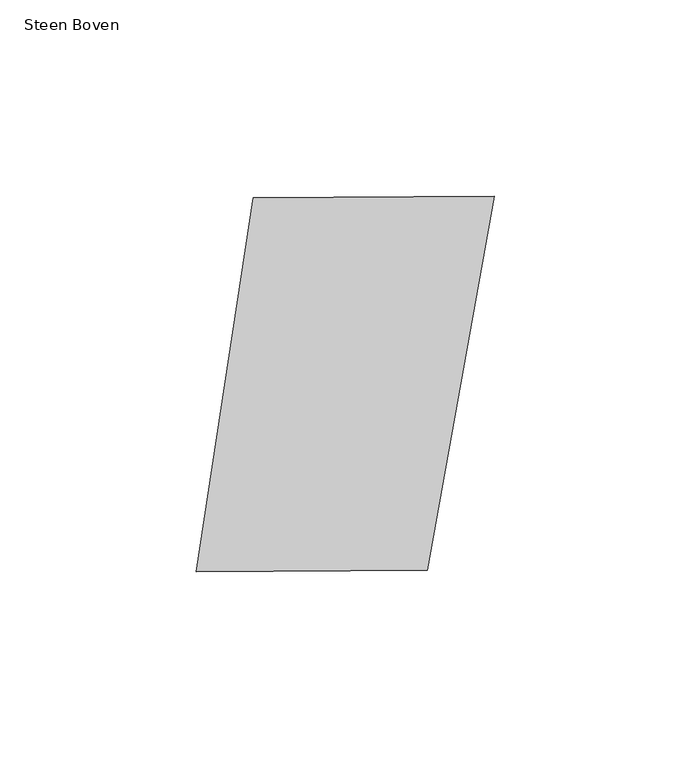
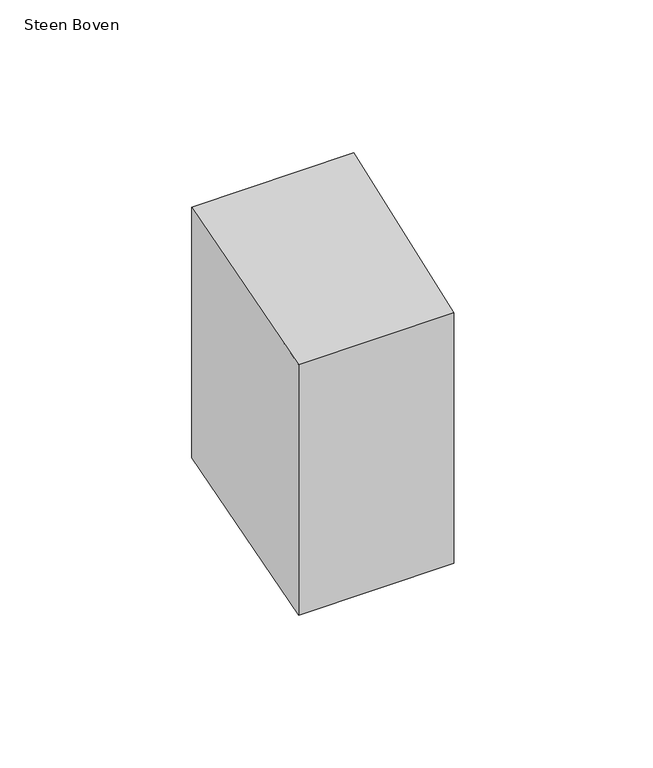
"""IFC4 building model written with IfcOpenShell, lengths in millimetres: proxy geometry, 00_GMA_steen_versie_4 : Steen Boven."""

from ifc_helpers import new_model, si_unit, origin, origin_with_axes, place, context, project, spatial, polyline, outline, extrude, source, transform, mapped, element, save


def steen_boven_38434019(model_context):
    return source(origin(), model_context, "Body", "SweptSolid", [
        extrude(outline(polyline([(109.568113, 118.6187659), (92.424621, 23.4422168), (33.7171718, 23.144437), (48.1404417, 118.28623), (109.568113, 118.6187659)])), origin_with_axes(), (0.0, 0.0, 1.0), 100.0),
    ])


if __name__ == "__main__":
    model = new_model("IFC4")
    model_context = context("Model", 3, world=origin())
    ifc_project = project(units=[si_unit("LENGTHUNIT", "METRE", prefix="MILLI")], contexts=[model_context])
    site = spatial("IfcSite", under=ifc_project)
    building = spatial("IfcBuilding", under=site)
    placement = place(None, origin())
    steen_boven_shape = steen_boven_38434019(model_context)
    element("IfcBuildingElementProxy", 1, Name="00_GMA_steen_versie_4 : Steen Boven", ObjectType="00_GMA_steen_versie_4 : Steen Boven", at=placement, inside=building, context=model_context, shape_type="MappedRepresentation", body=[
        mapped(steen_boven_shape, transform((0.0, 0.0, 0.0), x_axis=(1.0, 0.0, 0.0), y_axis=(0.0, 1.0, 0.0), z_axis=(0.0, 0.0, 1.0))),
    ])
    save(model, "model.ifc")

# Revit data of these elements
# Type "00_GMA_steen_versie_4 : Steen Boven"
#   StootVoegHalfBoven [instance default] = 5 mm
#   StootVoegHalf [instance default] = 5 mm
#   StootVoegBreedteOnder = 10 mm
#   StootVoegBreedteBoven = 10 mm
#   Steendikte = 100 mm
#   LintVoegOnderHalf = 5 mm
#   LintVoegOnder = 10 mm
#   LintVoegBovenHalf = 0 mm
#   LintVoegBoven = 0 mm
#   materiaal = none
#   MateriaalVoeg = none
#   Default Elevation = 0
